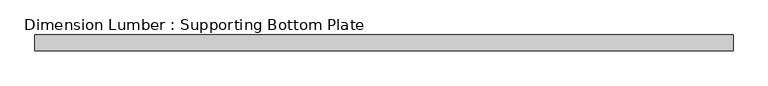
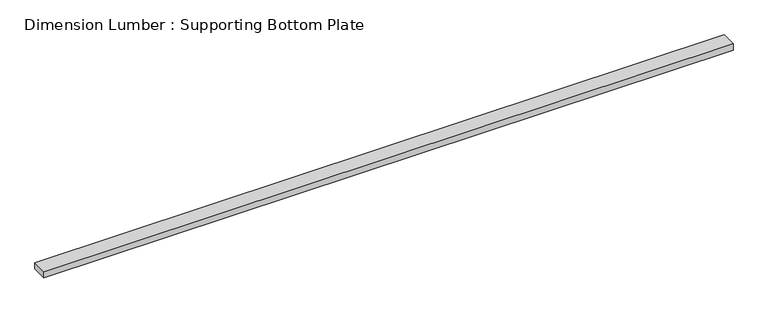
"""IFC4 building model written with IfcOpenShell, lengths in millimetres: beam geometry, Dimension Lumber : Supporting Bottom Plate."""

import ifcopenshell
import ifcopenshell.guid

model = None  # the IFC model being written
_history = None  # IfcOwnerHistory: only IFC2X3 demands one
_inside = {}  # id of a spatial element -> (the spatial element, [elements in it])
_under = {}  # id of a project, library or spatial element -> (it, [spatial elements below it])
_declared = {}  # id of a project -> (the project, [libraries it declares])
_typed = {}  # id of a type object -> (the type object, [elements of that type])
_made_of = {}  # id of a material, layer set ... -> (it, [elements and type objects made of it])


def new_model(schema):
    """Start an empty IFC model of exactly this schema.

    Asked for "IFC4X3", IfcOpenShell would pick the latest addendum, in which some entities
    have other attributes; the version numbers below select the first issue.
    IFC2X3 requires an IfcOwnerHistory on every rooted entity: one is made here for all.
    """
    global model, _history
    if schema == "IFC4X3":
        model = ifcopenshell.file(schema_version=(4, 3, 0, 0))
    else:
        model = ifcopenshell.file(schema=schema)
    _inside.clear()
    _under.clear()
    _declared.clear()
    _typed.clear()
    _made_of.clear()
    _history = None
    if model.schema == "IFC2X3":
        org = make("IfcOrganization", Name="unknown")
        user = make(
            "IfcPersonAndOrganization",
            ThePerson=make("IfcPerson", FamilyName="unknown"),
            TheOrganization=org,
        )
        app = make(
            "IfcApplication",
            ApplicationDeveloper=org,
            Version="unknown",
            ApplicationFullName="unknown",
            ApplicationIdentifier="unknown",
        )
        _history = make(
            "IfcOwnerHistory",
            OwningUser=user,
            OwningApplication=app,
            ChangeAction="ADDED",
            CreationDate=0,
        )
    return model


def make(cls, **values):
    """One entity of the class cls with the attributes given. An attribute that is None is left unset."""
    return model.create_entity(
        cls, **{name: value for name, value in values.items() if value is not None}
    )


def rooted(cls, **values):
    """An entity with a GlobalId (a new one), such as an element, a storey or a relation."""
    return make(cls, GlobalId=ifcopenshell.guid.new(), OwnerHistory=_history, **values)


def si_unit(unit_type, name, prefix=None):
    """IfcSIUnit, for example si_unit("LENGTHUNIT", "METRE", prefix="MILLI")."""
    return make("IfcSIUnit", UnitType=unit_type, Prefix=prefix, Name=name)


def assignment(units):
    """IfcUnitAssignment: the units of a project."""
    return None if units is None else make("IfcUnitAssignment", Units=units)


def point(xyz):
    """IfcCartesianPoint."""
    return None if xyz is None else make("IfcCartesianPoint", Coordinates=xyz)


def direction(xyz):
    """IfcDirection."""
    return None if xyz is None else make("IfcDirection", DirectionRatios=xyz)


def frame(location, z_axis=None, x_axis=None):
    """IfcAxis2Placement3D, a coordinate frame: its origin and axes. An axis left out is left unset."""
    return make(
        "IfcAxis2Placement3D",
        Location=point(location),
        Axis=direction(z_axis),
        RefDirection=direction(x_axis),
    )


def origin():
    """The frame at (0, 0, 0) with its axes left unset."""
    return frame((0.0, 0.0, 0.0))


def place(relative_to, where):
    """IfcLocalPlacement: puts the frame where relative to a parent placement (None: the world)."""
    return make(
        "IfcLocalPlacement", PlacementRelTo=relative_to, RelativePlacement=where
    )


def context(
    kind, dimensions, precision=None, world=None, true_north=None, identifier=None
):
    """IfcGeometricRepresentationContext, for example the 3D "Model" context."""
    return make(
        "IfcGeometricRepresentationContext",
        ContextIdentifier=identifier,
        ContextType=kind,
        CoordinateSpaceDimension=dimensions,
        Precision=precision,
        WorldCoordinateSystem=world,
        TrueNorth=true_north,
    )


def project(units=None, contexts=None):
    """IfcProject with its units and contexts."""
    return rooted(
        "IfcProject",
        Name="project",
        RepresentationContexts=contexts,
        UnitsInContext=assignment(units),
    )


def spatial(cls, under=None, at=None, **own):
    """A site, building, storey or space (cls), placed at a placement, below another one or the project."""
    s = rooted(cls, ObjectPlacement=at, **own)
    if under is not None:
        _under.setdefault(under.id(), (under, []))[1].append(s)
    return s


def polyline(points):
    """IfcPolyline through the points."""
    return make("IfcPolyline", Points=[point(p) for p in points])


def outline(outer, holes=None, kind="AREA"):
    """IfcArbitraryClosedProfileDef: a profile drawn as a closed curve; with holes, ...WithVoids."""
    if holes is None:
        return make("IfcArbitraryClosedProfileDef", ProfileType=kind, OuterCurve=outer)
    return make(
        "IfcArbitraryProfileDefWithVoids",
        ProfileType=kind,
        OuterCurve=outer,
        InnerCurves=holes,
    )


def extrude(swept, where, along, depth):
    """IfcExtrudedAreaSolid: the profile swept, set in the frame where, extruded along a direction by depth."""
    return make(
        "IfcExtrudedAreaSolid",
        SweptArea=swept,
        Position=where,
        ExtrudedDirection=direction(along),
        Depth=depth,
    )


def shape(context_of_items, identifier, shape_type, items):
    """IfcShapeRepresentation: the items that make up one representation, for example the "Body"."""
    return make(
        "IfcShapeRepresentation",
        ContextOfItems=context_of_items,
        RepresentationIdentifier=identifier,
        RepresentationType=shape_type,
        Items=items,
    )


def source(mapping_origin, context_of_items, identifier, shape_type, items):
    """IfcRepresentationMap: a shape defined once, which mapped items show again and again."""
    return make(
        "IfcRepresentationMap",
        MappingOrigin=mapping_origin,
        MappedRepresentation=shape(context_of_items, identifier, shape_type, items),
    )


def transform(
    local_origin,
    x_axis=None,
    y_axis=None,
    z_axis=None,
    scale=None,
    scale2=None,
    scale3=None,
    uniform=True,
):
    """IfcCartesianTransformationOperator3D, or its non-uniform kind. x_axis, y_axis, z_axis: its Axis1, 2, 3."""
    if uniform:
        return make(
            "IfcCartesianTransformationOperator3D",
            Axis1=direction(x_axis),
            Axis2=direction(y_axis),
            LocalOrigin=point(local_origin),
            Scale=scale,
            Axis3=direction(z_axis),
        )
    return make(
        "IfcCartesianTransformationOperator3DnonUniform",
        Axis1=direction(x_axis),
        Axis2=direction(y_axis),
        LocalOrigin=point(local_origin),
        Scale=scale,
        Axis3=direction(z_axis),
        Scale2=scale2,
        Scale3=scale3,
    )


def mapped(mapping_source, mapping_target):
    """IfcMappedItem: shows the shape of a source again, moved by a transform."""
    return make(
        "IfcMappedItem", MappingSource=mapping_source, MappingTarget=mapping_target
    )


def made_of(thing, what):
    """Note that an element or type object is made of a material, layer set ...; save() writes the relation."""
    if what is not None:
        _made_of.setdefault(what.id(), (what, []))[1].append(thing)
    return thing


def element(
    cls,
    number,
    at=None,
    inside=None,
    cuts=None,
    type_object=None,
    material=None,
    context=None,
    identifier="Body",
    shape_type=None,
    held_by="IfcProductDefinitionShape",
    body=None,
    shapes=None,
    **own,
):
    """One element of the class cls, such as IfcWall. Its Tag is "e" and its number.

    at: its placement. inside: the storey or other place that contains it. cuts: it is an
    opening in that element (IfcRelVoidsElement). A single representation is given by context,
    identifier, shape_type and body (its items); several are given by shapes. held_by: the class
    of the entity that holds the representations. save() writes the other relations.
    """
    e = rooted(cls, Tag="e%d" % number, ObjectPlacement=at, **own)
    if body is not None:
        shapes = [shape(context, identifier, shape_type, body)]
    if shapes is not None:
        e.Representation = make(held_by, Representations=shapes)
    if inside is not None:
        _inside.setdefault(inside.id(), (inside, []))[1].append(e)
    if cuts is not None:
        rooted(
            "IfcRelVoidsElement", RelatingBuildingElement=cuts, RelatedOpeningElement=e
        )
    if type_object is not None:
        _typed.setdefault(type_object.id(), (type_object, []))[1].append(e)
    return made_of(e, material)


def aggregate(whole, parts):
    """IfcRelAggregates: a whole, such as a stair, and the parts it consists of."""
    return rooted("IfcRelAggregates", RelatingObject=whole, RelatedObjects=parts)


def save(model, path):
    """Write the relations noted so far, then the file.

    IfcRelAggregates (storeys below a building ...), IfcRelContainedInSpatialStructure (elements
    in a storey), IfcRelDefinesByType, IfcRelAssociatesMaterial and IfcRelDeclares: one each for
    every whole, place, type object, material and project.
    """
    for whole, parts in _under.values():
        aggregate(whole, parts)
    for where, things in _inside.values():
        rooted(
            "IfcRelContainedInSpatialStructure",
            RelatedElements=things,
            RelatingStructure=where,
        )
    for kind, things in _typed.values():
        rooted("IfcRelDefinesByType", RelatedObjects=things, RelatingType=kind)
    for what, things in _made_of.values():
        rooted("IfcRelAssociatesMaterial", RelatedObjects=things, RelatingMaterial=what)
    for by, libraries in _declared.values():
        rooted("IfcRelDeclares", RelatingContext=by, RelatedDefinitions=libraries)
    model.write(path)


def dimension_lumber_supporting_bottom_plate_14fdda6b(model_context):
    return source(origin(), model_context, "Body", "SweptSolid", [
        extrude(outline(polyline([(1910.55625, 44.45), (1910.55625, -44.45), (-1999.45625, -44.45), (-1999.45625, 44.45), (1910.55625, 44.45)])), frame((0.0, 0.0, -19.05), z_axis=(0.0, 0.0, 1.0), x_axis=(1.0, 0.0, 0.0)), (0.0, 0.0, 1.0), 38.1),
    ])


if __name__ == "__main__":
    model = new_model("IFC4")
    model_context = context("Model", 3, world=origin())
    ifc_project = project(units=[si_unit("LENGTHUNIT", "METRE", prefix="MILLI")], contexts=[model_context])
    site = spatial("IfcSite", under=ifc_project)
    building = spatial("IfcBuilding", under=site)
    placement = place(None, origin())
    dimension_lumber_supporting_bottom_plate_shape = dimension_lumber_supporting_bottom_plate_14fdda6b(model_context)
    element("IfcBeam", 1, ObjectType="Dimension Lumber : Supporting Bottom Plate", at=placement, inside=building, context=model_context, shape_type="MappedRepresentation", body=[
        mapped(dimension_lumber_supporting_bottom_plate_shape, transform((0.0, 0.0, 0.0), x_axis=(1.0, 0.0, 0.0), y_axis=(0.0, 1.0, 0.0), z_axis=(0.0, 0.0, 1.0))),
    ])
    save(model, "model.ifc")

# Revit data of these elements
# Type "Dimension Lumber : Supporting Bottom Plate"
#   Assembly Code = "B10"
#   A = 0.0364583 SF
#   Length [instance default] = 5' - 0"
#   b = 0' - 3 1/2"
#   d = 0' - 1 1/2"
#   Structural Material [instance default] = Softwood, Lumber
# Element 1 (IfcBeam, "Dimension Lumber : Supporting Bottom Plate")
#   Structural Material = Douglas Fir #2
#   Materials on its faces: "Douglas Fir #2"
# Materials
#   "Softwood, Lumber": class "Wood", colour RGB 223 192 134, transparency 0, Description = "Pinus Echinata", Cost = 0
#   "Douglas Fir #2": class "Wood", colour RGB 223 192 134, transparency 0, Description = "Pinus Echinata", Cost = 0
